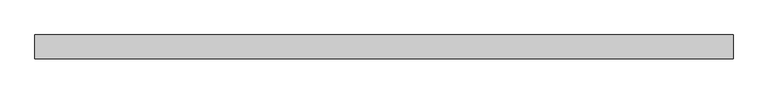
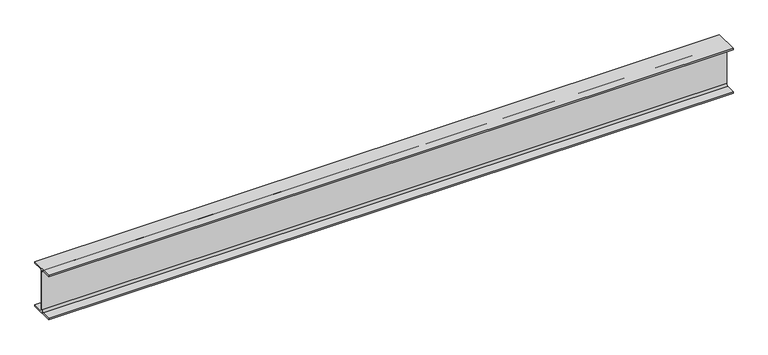
"""IFC4 building model written with IfcOpenShell, lengths in millimetres: beam geometry, 0912_Steel Framing_H-KSD3502 : H_SB_ASB_H-400x200x8x13."""

from ifc_helpers import new_model, si_unit, point, frame, frame_2d, origin, place, context, project, spatial, polyline, circle_curve, trimmed, segment, composite_curve, outline, extrude, source, transform, mapped, element, save


def beam_b18b0c5b(model_context):
    return source(origin(), model_context, "Body", "SweptSolid", [
        extrude(outline(composite_curve([segment(polyline([(100.0, -187.0), (100.0, -200.0), (-100.0, -200.0), (-100.0, -187.0), (-20.0, -187.0)]), True, "CONTINUOUS"), segment(trimmed(circle_curve(frame_2d((-20.0, -171.0)), 16.0), [point((-20.0, -187.0))], [point((-4.0, -171.0))], True, "CARTESIAN"), True, "CONTINUOUS"), segment(polyline([(-4.0, -171.0), (-4.0, 171.0)]), True, "CONTINUOUS"), segment(trimmed(circle_curve(frame_2d((-20.0, 171.0)), 16.0), [point((-4.0, 171.0))], [point((-20.0, 187.0))], True, "CARTESIAN"), True, "CONTINUOUS"), segment(polyline([(-20.0, 187.0), (-100.0, 187.0), (-100.0, 200.0), (100.0, 200.0), (100.0, 187.0), (20.0, 187.0)]), True, "CONTINUOUS"), segment(trimmed(circle_curve(frame_2d((20.0, 171.0)), 16.0), [point((20.0, 187.0))], [point((4.0, 171.0))], True, "CARTESIAN"), True, "CONTINUOUS"), segment(polyline([(4.0, 171.0), (4.0, -171.0)]), True, "CONTINUOUS"), segment(trimmed(circle_curve(frame_2d((20.0, -171.0)), 16.0), [point((4.0, -171.0))], [point((20.0, -187.0))], True, "CARTESIAN"), True, "CONTINUOUS"), segment(polyline([(20.0, -187.0), (100.0, -187.0)]), True, "CONTINUOUS")], self_intersect=False)), frame((-2904.8, 0.0, 0.0), z_axis=(1.0, 0.0, 0.0), x_axis=(0.0, 1.0, 0.0)), (0.0, 0.0, 1.0), 5809.6),
    ])


if __name__ == "__main__":
    model = new_model("IFC4")
    model_context = context("Model", 3, world=origin())
    ifc_project = project(units=[si_unit("LENGTHUNIT", "METRE", prefix="MILLI")], contexts=[model_context])
    site = spatial("IfcSite", under=ifc_project)
    building = spatial("IfcBuilding", under=site)
    placement = place(None, origin())
    beam_shape = beam_b18b0c5b(model_context)
    element("IfcBeam", 1, ObjectType="0912_Steel Framing_H-KSD3502 : H_SB_ASB_H-400x200x8x13", at=placement, inside=building, context=model_context, shape_type="MappedRepresentation", body=[
        mapped(beam_shape, transform((0.0, 0.0, 0.0), x_axis=(1.0, 0.0, 0.0), y_axis=(0.0, 1.0, 0.0), z_axis=(0.0, 0.0, 1.0))),
    ])
    save(model, "model.ifc")

# Revit data of these elements
# Type "0912_Steel Framing_H-KSD3502 : H_SB_ASB_H-400x200x8x13"
#   H_WM Code_1 = "S01AA002-00001 | Main Steel Structure Fabrication Work | Shelter/Building | Medium Steel - Standard (90KG/M>Weight≥30KG/M) | Material: (   )"
#   H_WM Code_2 = "S03AA028-00001 | Main Steel Structure Erection Work | Shelter/Building | Medium Steel (90KG/M>Weight≥30KG/M) | Material: (   )"
#   H_WM Code_3 = "S01AA010-00001 | Main Steel Structure Fabrication Work | Shelter/Building | Steel Painting/Coating | for Non-Fireproofed Steel Surface, Surface Preparation, Primer, Second & Final Coat | Material: (   )"
#   H_Q'ty Cal Type Tag = "SB-Q2"
#   Width = 20.0 cm
#   Web Thickness = 0.8 cm
#   Web Fillet = 1.6 cm
#   Warping Constant = 649000.0 cm⁶
#   W = 0
#   Torsional Moment of Inertia = 35.8981 cm⁴
#   Section Area = 84.12 cm²
#   Plastic Modulus weak axis = 268.0 cm³
#   Plastic Modulus strong axis = 1330.0 cm³
#   Perimeter = 1.56 m²/m
#   Nominal Weight = 66.00 kgf/m
#   Moment of Inertia weak axis = 1740.00 cm⁴
#   Moment of Inertia strong axis = 23700.00 cm⁴
#   Height = 40.0 cm
#   Flange Thickness = 1.3 cm
#   Elastic Modulus weak axis = 174.0 cm³
#   Elastic Modulus strong axis = 1190.0 cm³
#   Centroid Vertical = 20.0 cm
#   Centroid Horizontal = 10.0 cm
#   Ix = 237000000
#   Length [instance default] = 1.5240 m
#   Zx = 1330000
#   b = 0.2000 m
#   h = 0.4000 m
#   r = 0.0160 m
#   s = 0.0080 m
#   t = 0.0130 m
#   A = 0.008412 m²
#   Structural Material [instance default] = Steel, 45-345
#   Assembly Code = ""
# Element 1 (IfcBeam, "0912_Steel Framing_H-KSD3502 : H_SB_ASB_H-400x200x8x13")
#   Structural Material = none
# Materials
#   "Steel, 45-345": class "Metal", colour RGB 189 187 185, transparency 0, Description = "Steel 345 MPa", Cost = 0
